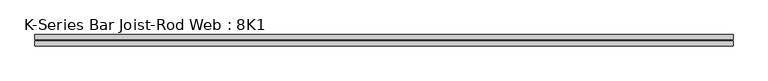
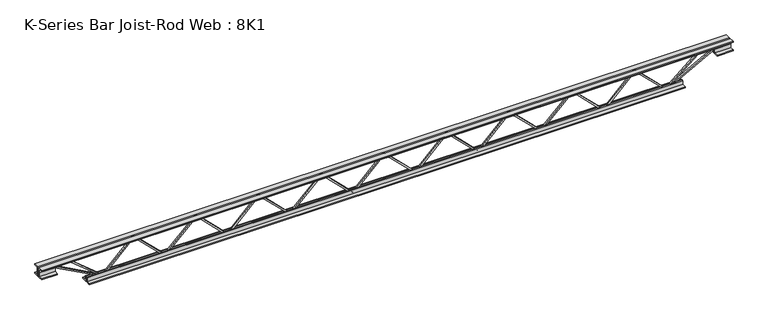
"""IFC4 building model written with IfcOpenShell, lengths in millimetres: beam geometry, K-Series Bar Joist-Rod Web : 8K1."""

from ifc_helpers import new_model, si_unit, frame, origin, place, context, project, spatial, polyline, outline, extrude, source, transform, mapped, element, save


def k_series_bar_joist_rod_web_8k1_857b1893(model_context):
    return source(origin(), model_context, "Body", "SweptSolid", [
        extrude(outline(polyline([(-90.4875, 997.1394773), (-100.0125, 997.1394773), (-100.0125, 1002.2684463), (90.4875, 1195.3463418), (90.4875, 1197.7884038), (-100.0125, 1390.8662992), (-100.0125, 1395.9952683), (-90.4875, 1395.9952683), (-90.4875, 1394.7742373), (100.0125, 1201.6963418), (100.0125, 1191.4384038), (-90.4875, 998.3605083), (-90.4875, 997.1394773)])), frame((0.0, -4.7625, 0.0), z_axis=(0.0, 1.0, 0.0), x_axis=(0.0, 0.0, 1.0)), (0.0, 0.0, 1.0), 9.525),
        extrude(outline(polyline([(-90.4875, 598.2836864), (-100.0125, 598.2836864), (-100.0125, 603.4126554), (90.4875, 796.4905509), (90.4875, 798.9326128), (-100.0125, 992.0105083), (-100.0125, 997.1394773), (-90.4875, 997.1394773), (-90.4875, 995.9184463), (100.0125, 802.8405509), (100.0125, 792.5826128), (-90.4875, 599.5047174), (-90.4875, 598.2836864)])), frame((0.0, -4.7625, 0.0), z_axis=(0.0, 1.0, 0.0), x_axis=(0.0, 0.0, 1.0)), (0.0, 0.0, 1.0), 9.525),
        extrude(outline(polyline([(-90.4875, 199.4278955), (-100.0125, 199.4278955), (-100.0125, 204.5568645), (90.4875, 397.63476), (90.4875, 400.0768219), (-100.0125, 593.1547174), (-100.0125, 598.2836864), (-90.4875, 598.2836864), (-90.4875, 597.0626554), (100.0125, 403.98476), (100.0125, 393.7268219), (-90.4875, 200.6489264), (-90.4875, 199.4278955)])), frame((0.0, -4.7625, 0.0), z_axis=(0.0, 1.0, 0.0), x_axis=(0.0, 0.0, 1.0)), (0.0, 0.0, 1.0), 9.525),
        extrude(outline(polyline([(-90.4875, -199.4278955), (-100.0125, -199.4278955), (-100.0125, -194.2989264), (90.4875, -1.221031), (90.4875, 1.221031), (-100.0125, 194.2989264), (-100.0125, 199.4278955), (-90.4875, 199.4278955), (-90.4875, 198.2068645), (100.0125, 5.128969), (100.0125, -5.128969), (-90.4875, -198.2068645), (-90.4875, -199.4278955)])), frame((0.0, -4.7625, 0.0), z_axis=(0.0, 1.0, 0.0), x_axis=(0.0, 0.0, 1.0)), (0.0, 0.0, 1.0), 9.525),
        extrude(outline(polyline([(-90.4875, -598.2836864), (-100.0125, -598.2836864), (-100.0125, -593.1547174), (90.4875, -400.0768219), (90.4875, -397.63476), (-100.0125, -204.5568645), (-100.0125, -199.4278955), (-90.4875, -199.4278955), (-90.4875, -200.6489264), (100.0125, -393.7268219), (100.0125, -403.98476), (-90.4875, -597.0626554), (-90.4875, -598.2836864)])), frame((0.0, -4.7625, 0.0), z_axis=(0.0, 1.0, 0.0), x_axis=(0.0, 0.0, 1.0)), (0.0, 0.0, 1.0), 9.525),
        extrude(outline(polyline([(-90.4875, -997.1394773), (-100.0125, -997.1394773), (-100.0125, -992.0105083), (90.4875, -798.9326128), (90.4875, -796.4905509), (-100.0125, -603.4126554), (-100.0125, -598.2836864), (-90.4875, -598.2836864), (-90.4875, -599.5047174), (100.0125, -792.5826128), (100.0125, -802.8405509), (-90.4875, -995.9184463), (-90.4875, -997.1394773)])), frame((0.0, -4.7625, 0.0), z_axis=(0.0, 1.0, 0.0), x_axis=(0.0, 0.0, 1.0)), (0.0, 0.0, 1.0), 9.525),
        extrude(outline(polyline([(-90.4875, -1395.9952683), (-100.0125, -1395.9952683), (-100.0125, -1390.8662992), (90.4875, -1197.7884038), (90.4875, -1195.3463418), (-100.0125, -1002.2684463), (-100.0125, -997.1394773), (-90.4875, -997.1394773), (-90.4875, -998.3605083), (100.0125, -1191.4384038), (100.0125, -1201.6963418), (-90.4875, -1394.7742373), (-90.4875, -1395.9952683)])), frame((0.0, -4.7625, 0.0), z_axis=(0.0, 1.0, 0.0), x_axis=(0.0, 0.0, 1.0)), (0.0, 0.0, 1.0), 9.525),
        extrude(outline(polyline([(-90.4875, 1395.9952683), (-100.0125, 1395.9952683), (-100.0125, 1401.1242373), (90.4875, 1594.2021327), (90.4875, 1596.6441947), (-100.0125, 1789.7220902), (-100.0125, 1794.8510592), (-90.4875, 1794.8510592), (-90.4875, 1793.6300282), (100.0125, 1600.5521327), (100.0125, 1590.2941947), (-90.4875, 1397.2162992), (-90.4875, 1395.9952683)])), frame((0.0, -4.7625, 0.0), z_axis=(0.0, 1.0, 0.0), x_axis=(0.0, 0.0, 1.0)), (0.0, 0.0, 1.0), 9.525),
        extrude(outline(polyline([(-90.4875, -1794.8510592), (-100.0125, -1794.8510592), (-100.0125, -1789.7220902), (90.4875, -1596.6441947), (90.4875, -1594.2021327), (-100.0125, -1401.1242373), (-100.0125, -1395.9952683), (-90.4875, -1395.9952683), (-90.4875, -1397.2162992), (100.0125, -1590.2941947), (100.0125, -1600.5521327), (-90.4875, -1793.6300282), (-90.4875, -1794.8510592)])), frame((0.0, -4.7625, 0.0), z_axis=(0.0, 1.0, 0.0), x_axis=(0.0, 0.0, 1.0)), (0.0, 0.0, 1.0), 9.525),
        extrude(outline(polyline([(4.7625, 101.6), (36.5125, 101.6), (36.5125, 95.25), (11.1125, 95.25), (11.1125, 69.85), (4.7625, 69.85), (4.7625, 101.6)])), frame((-2201.2510592, 0.0, 0.0), z_axis=(1.0, 0.0, 0.0), x_axis=(0.0, 1.0, 0.0)), (0.0, 0.0, 1.0), 4402.5021184),
        extrude(outline(polyline([(-4.7625, 101.6), (-4.7625, 69.85), (-11.1125, 69.85), (-11.1125, 95.25), (-36.5125, 95.25), (-36.5125, 101.6), (-4.7625, 101.6)])), frame((-2201.2510592, 0.0, 0.0), z_axis=(1.0, 0.0, 0.0), x_axis=(0.0, 1.0, 0.0)), (0.0, 0.0, 1.0), 4402.5021184),
        extrude(outline(polyline([(-4.7625, 38.1), (-36.5125, 38.1), (-36.5125, 44.45), (-11.1125, 44.45), (-11.1125, 69.85), (-4.7625, 69.85), (-4.7625, 38.1)])), frame((-2201.2510592, 0.0, 0.0), z_axis=(1.0, 0.0, 0.0), x_axis=(0.0, 1.0, 0.0)), (0.0, 0.0, 1.0), 101.6),
        extrude(outline(polyline([(36.5125, 38.1), (4.7625, 38.1), (4.7625, 69.85), (11.1125, 69.85), (11.1125, 44.45), (36.5125, 44.45), (36.5125, 38.1)])), frame((-2201.2510592, 0.0, 0.0), z_axis=(1.0, 0.0, 0.0), x_axis=(0.0, 1.0, 0.0)), (0.0, 0.0, 1.0), 101.6),
        extrude(outline(polyline([(4.7625, 38.1), (4.7625, 69.85), (11.1125, 69.85), (11.1125, 44.45), (36.5125, 44.45), (36.5125, 38.1), (4.7625, 38.1)])), frame((2099.6510592, 0.0, 0.0), z_axis=(1.0, 0.0, 0.0), x_axis=(0.0, 1.0, 0.0)), (0.0, 0.0, 1.0), 101.6),
        extrude(outline(polyline([(-4.7625, 38.1), (-36.5125, 38.1), (-36.5125, 44.45), (-11.1125, 44.45), (-11.1125, 69.85), (-4.7625, 69.85), (-4.7625, 38.1)])), frame((2099.6510592, 0.0, 0.0), z_axis=(1.0, 0.0, 0.0), x_axis=(0.0, 1.0, 0.0)), (0.0, 0.0, 1.0), 101.6),
        extrude(outline(polyline([(4.7625, -101.6), (4.7625, -69.85), (11.1125, -69.85), (11.1125, -95.25), (36.5125, -95.25), (36.5125, -101.6), (4.7625, -101.6)])), frame((-1896.4510592, 0.0, 0.0), z_axis=(1.0, 0.0, 0.0), x_axis=(0.0, 1.0, 0.0)), (0.0, 0.0, 1.0), 3792.9021184),
        extrude(outline(polyline([(-4.7625, -101.6), (-36.5125, -101.6), (-36.5125, -95.25), (-11.1125, -95.25), (-11.1125, -69.85), (-4.7625, -69.85), (-4.7625, -101.6)])), frame((-1896.4510592, 0.0, 0.0), z_axis=(1.0, 0.0, 0.0), x_axis=(0.0, 1.0, 0.0)), (0.0, 0.0, 1.0), 3792.9021184),
        extrude(outline(polyline([(0.0, -9.525), (0.0, 0.0), (346.6425392, 0.0), (346.6425392, -9.525), (0.0, -9.525)])), frame((-2101.9193577, 4.7625, 65.662372), z_axis=(0.4762831485400805, 0.0, 0.8792919665371381), x_axis=(0.8792919665371381, 0.0, -0.4762831485400805)), (0.0, 0.0, 1.0), 9.525),
        extrude(outline(polyline([(0.0, -9.525), (0.0, 0.0), (258.9005514, 0.0), (258.9005514, -9.525), (0.0, -9.525)])), frame((-1997.3159847, 4.7625, 66.1815051), z_axis=(0.637696594843947, 0.0, 0.770287642977891), x_axis=(0.770287642977891, 0.0, -0.637696594843947)), (0.0, 0.0, 1.0), 9.525),
        extrude(outline(polyline([(0.0, -9.525), (0.0, 0.0), (346.6425392, 0.0), (346.6425392, -9.525), (0.0, -9.525)])), frame((2101.9193577, -4.7625, 65.662372), z_axis=(-0.47628314854004083, 0.0, 0.8792919665371597), x_axis=(-0.8792919665371597, 0.0, -0.47628314854004083)), (0.0, 0.0, 1.0), 9.525),
        extrude(outline(polyline([(0.0, -9.525), (0.0, 0.0), (258.9005514, 0.0), (258.9005514, -9.525), (0.0, -9.525)])), frame((1997.3159847, -4.7625, 66.1815051), z_axis=(-0.6376965948439217, 0.0, 0.770287642977912), x_axis=(-0.770287642977912, 0.0, -0.6376965948439217)), (0.0, 0.0, 1.0), 9.525),
    ])


if __name__ == "__main__":
    model = new_model("IFC4")
    model_context = context("Model", 3, world=origin())
    ifc_project = project(units=[si_unit("LENGTHUNIT", "METRE", prefix="MILLI")], contexts=[model_context])
    site = spatial("IfcSite", under=ifc_project)
    building = spatial("IfcBuilding", under=site)
    placement = place(None, origin())
    k_series_bar_joist_rod_web_8k1_shape = k_series_bar_joist_rod_web_8k1_857b1893(model_context)
    element("IfcBeam", 1, ObjectType="K-Series Bar Joist-Rod Web : 8K1", at=placement, inside=building, context=model_context, shape_type="MappedRepresentation", body=[
        mapped(k_series_bar_joist_rod_web_8k1_shape, transform((0.0, 0.0, 0.0), x_axis=(1.0, 0.0, 0.0), y_axis=(0.0, 1.0, 0.0), z_axis=(0.0, 0.0, 1.0))),
    ])
    save(model, "model.ifc")

# Revit data of these elements
# Type "K-Series Bar Joist-Rod Web : 8K1"
#   Assembly Code = "B1010350"
#   Wt = 5.1
#   Web Thickness = 0' - 0 3/8"
#   Start Offset [instance default] = 0' - 0"
#   Start Extension [instance default] = 0' - 0"
#   Seat Length = 0' - 4"
#   Seat Depth = 0' - 2 1/2"
#   PanelArrayLength [instance default] = 21' - 4"
#   Panel [instance default] = 1' - 4"
#   End Offset [instance default] = 0' - 0"
#   End Extension [instance default] = 0' - 0"
#   End Panel = 1' - 4"
#   Cord Leg = 0' - 1 1/4"
#   Chord Thickness = 0' - 0 1/4"
#   Length [instance default] = 24' - 0"
#   Depth = 0' - 8"
#   PanelArrayNum [instance default] = 16
#   Rendering Material = none
# Element 1 (IfcBeam, "K-Series Bar Joist-Rod Web : 8K1")
#   PanelArrayLength = 11' - 9.32686"
#   Panel = 1' - 3.70298"
#   PanelArrayNum = 9
